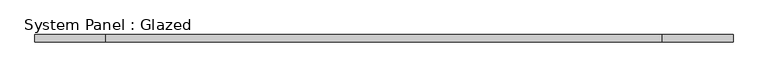
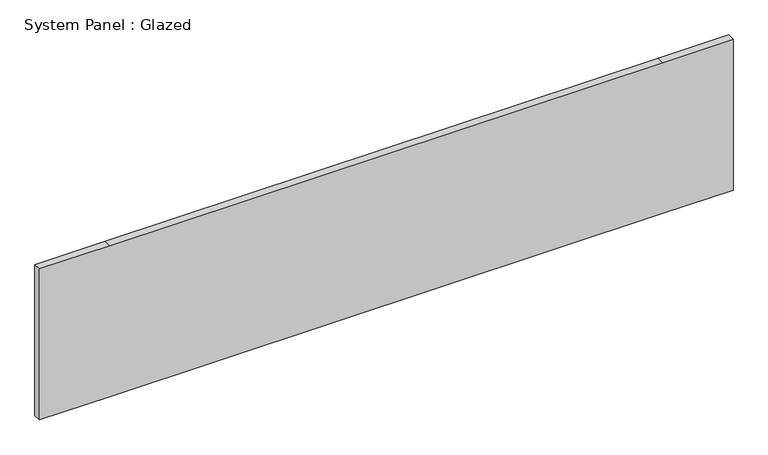
"""IFC4 building model written with IfcOpenShell, lengths in millimetres: plate geometry, System Panel : Glazed."""

from ifc_helpers import new_model, si_unit, frame, origin, place, context, project, spatial, polyline, outline, extrude, source, transform, mapped, element, save


def system_panel_glazed_7ab8f380(model_context):
    return source(origin(), model_context, "Body", "SweptSolid", [
        extrude(outline(polyline([(0.0, -1187.45), (0.0, -946.15), (0.0, 946.15), (0.0, 1187.45), (546.1, 1187.45), (546.1, 946.15), (546.1, -946.15), (546.1, -1187.45), (0.0, -1187.45)])), frame((0.0, -44.45, 0.0), z_axis=(0.0, 1.0, 0.0), x_axis=(0.0, 0.0, 1.0)), (0.0, 0.0, 1.0), 25.4),
    ])


if __name__ == "__main__":
    model = new_model("IFC4")
    model_context = context("Model", 3, world=origin())
    ifc_project = project(units=[si_unit("LENGTHUNIT", "METRE", prefix="MILLI")], contexts=[model_context])
    site = spatial("IfcSite", under=ifc_project)
    building = spatial("IfcBuilding", under=site)
    placement = place(None, origin())
    system_panel_glazed_shape = system_panel_glazed_7ab8f380(model_context)
    element("IfcPlate", 1, ObjectType="System Panel : Glazed", at=placement, inside=building, context=model_context, shape_type="MappedRepresentation", body=[
        mapped(system_panel_glazed_shape, transform((0.0, 0.0, 0.0), x_axis=(1.0, 0.0, 0.0), y_axis=(0.0, 1.0, 0.0), z_axis=(0.0, 0.0, 1.0))),
    ])
    save(model, "model.ifc")

# Revit data of these elements
# Element 1 (IfcPlate, "System Panel : Glazed")
#   Materials on its faces: "Glass"
# Materials
#   "Glass": class "Glass", colour RGB 0 128 192, transparency 0.75, Cost = 0
